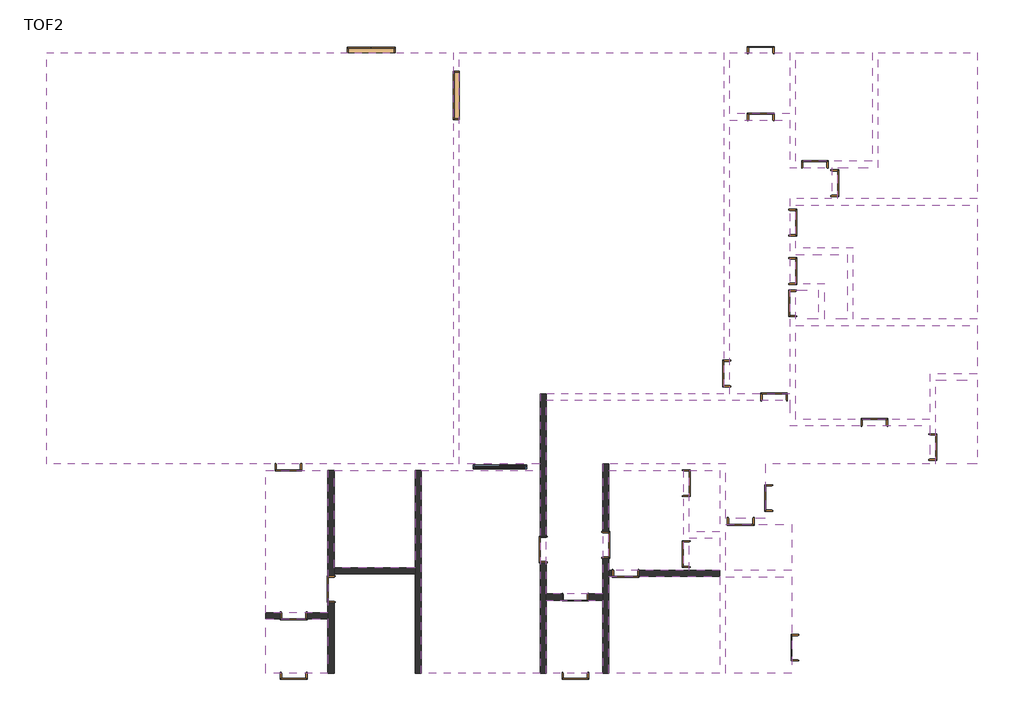
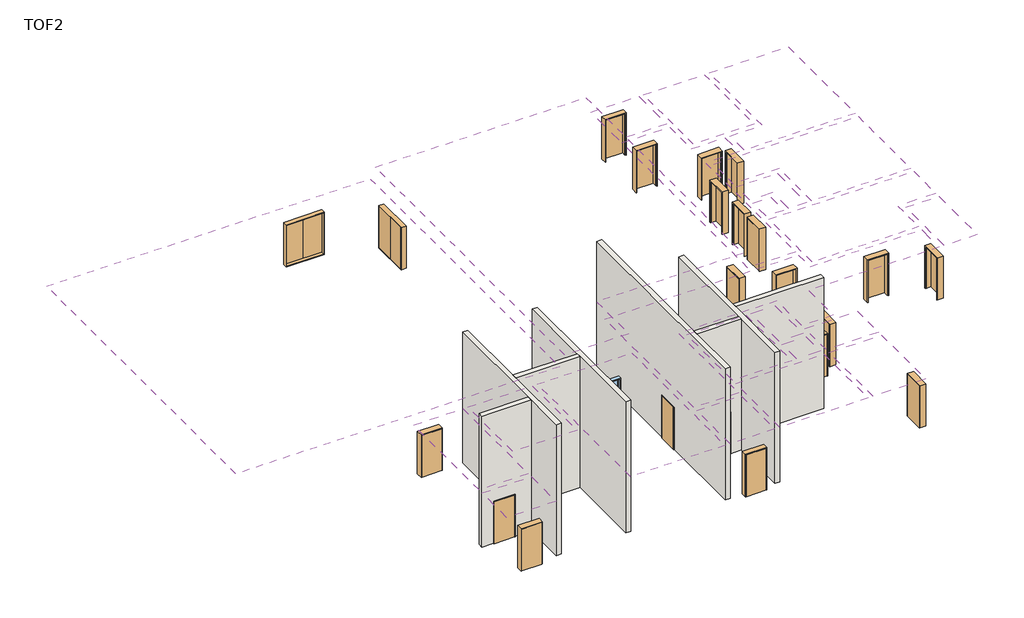
# One storey: 27 doors, 23 coverings, 8 walls, 1 window.
"""IFC4 building model written with IfcOpenShell, lengths in millimetres."""

import ifcopenshell
import ifcopenshell.guid

model = None  # the IFC model being written
_history = None  # IfcOwnerHistory: only IFC2X3 demands one
_inside = {}  # id of a spatial element -> (the spatial element, [elements in it])
_under = {}  # id of a project, library or spatial element -> (it, [spatial elements below it])
_declared = {}  # id of a project -> (the project, [libraries it declares])
_typed = {}  # id of a type object -> (the type object, [elements of that type])
_made_of = {}  # id of a material, layer set ... -> (it, [elements and type objects made of it])


def new_model(schema):
    """Start an empty IFC model of exactly this schema.

    Asked for "IFC4X3", IfcOpenShell would pick the latest addendum, in which some entities
    have other attributes; the version numbers below select the first issue.
    IFC2X3 requires an IfcOwnerHistory on every rooted entity: one is made here for all.
    """
    global model, _history
    if schema == "IFC4X3":
        model = ifcopenshell.file(schema_version=(4, 3, 0, 0))
    else:
        model = ifcopenshell.file(schema=schema)
    _inside.clear()
    _under.clear()
    _declared.clear()
    _typed.clear()
    _made_of.clear()
    _history = None
    if model.schema == "IFC2X3":
        org = make("IfcOrganization", Name="unknown")
        user = make(
            "IfcPersonAndOrganization",
            ThePerson=make("IfcPerson", FamilyName="unknown"),
            TheOrganization=org,
        )
        app = make(
            "IfcApplication",
            ApplicationDeveloper=org,
            Version="unknown",
            ApplicationFullName="unknown",
            ApplicationIdentifier="unknown",
        )
        _history = make(
            "IfcOwnerHistory",
            OwningUser=user,
            OwningApplication=app,
            ChangeAction="ADDED",
            CreationDate=0,
        )
    return model


def make(cls, **values):
    """One entity of the class cls with the attributes given. An attribute that is None is left unset."""
    return model.create_entity(
        cls, **{name: value for name, value in values.items() if value is not None}
    )


def rooted(cls, **values):
    """An entity with a GlobalId (a new one), such as an element, a storey or a relation."""
    return make(cls, GlobalId=ifcopenshell.guid.new(), OwnerHistory=_history, **values)


def si_unit(unit_type, name, prefix=None):
    """IfcSIUnit, for example si_unit("LENGTHUNIT", "METRE", prefix="MILLI")."""
    return make("IfcSIUnit", UnitType=unit_type, Prefix=prefix, Name=name)


def assignment(units):
    """IfcUnitAssignment: the units of a project."""
    return None if units is None else make("IfcUnitAssignment", Units=units)


def point(xyz):
    """IfcCartesianPoint."""
    return None if xyz is None else make("IfcCartesianPoint", Coordinates=xyz)


def direction(xyz):
    """IfcDirection."""
    return None if xyz is None else make("IfcDirection", DirectionRatios=xyz)


def frame(location, z_axis=None, x_axis=None):
    """IfcAxis2Placement3D, a coordinate frame: its origin and axes. An axis left out is left unset."""
    return make(
        "IfcAxis2Placement3D",
        Location=point(location),
        Axis=direction(z_axis),
        RefDirection=direction(x_axis),
    )


def origin():
    """The frame at (0, 0, 0) with its axes left unset."""
    return frame((0.0, 0.0, 0.0))


def origin_with_axes():
    """The frame at (0, 0, 0) with the z axis (0, 0, 1) and the x axis (1, 0, 0) written out."""
    return frame((0.0, 0.0, 0.0), z_axis=(0.0, 0.0, 1.0), x_axis=(1.0, 0.0, 0.0))


def place(relative_to, where):
    """IfcLocalPlacement: puts the frame where relative to a parent placement (None: the world)."""
    return make(
        "IfcLocalPlacement", PlacementRelTo=relative_to, RelativePlacement=where
    )


def context(
    kind, dimensions, precision=None, world=None, true_north=None, identifier=None
):
    """IfcGeometricRepresentationContext, for example the 3D "Model" context."""
    return make(
        "IfcGeometricRepresentationContext",
        ContextIdentifier=identifier,
        ContextType=kind,
        CoordinateSpaceDimension=dimensions,
        Precision=precision,
        WorldCoordinateSystem=world,
        TrueNorth=true_north,
    )


def project(units=None, contexts=None):
    """IfcProject with its units and contexts."""
    return rooted(
        "IfcProject",
        Name="project",
        RepresentationContexts=contexts,
        UnitsInContext=assignment(units),
    )


def spatial(cls, under=None, at=None, **own):
    """A site, building, storey or space (cls), placed at a placement, below another one or the project."""
    s = rooted(cls, ObjectPlacement=at, **own)
    if under is not None:
        _under.setdefault(under.id(), (under, []))[1].append(s)
    return s


def polyline(points):
    """IfcPolyline through the points."""
    return make("IfcPolyline", Points=[point(p) for p in points])


def outline(outer, holes=None, kind="AREA"):
    """IfcArbitraryClosedProfileDef: a profile drawn as a closed curve; with holes, ...WithVoids."""
    if holes is None:
        return make("IfcArbitraryClosedProfileDef", ProfileType=kind, OuterCurve=outer)
    return make(
        "IfcArbitraryProfileDefWithVoids",
        ProfileType=kind,
        OuterCurve=outer,
        InnerCurves=holes,
    )


def extrude(swept, where, along, depth):
    """IfcExtrudedAreaSolid: the profile swept, set in the frame where, extruded along a direction by depth."""
    return make(
        "IfcExtrudedAreaSolid",
        SweptArea=swept,
        Position=where,
        ExtrudedDirection=direction(along),
        Depth=depth,
    )


def faces_of(points, faces, orient=None, outer=None):
    """IfcFace entities. A face is a list of loops; a loop is a list of indices into points, from 0.

    orient and outer hold one flag for each loop. By default every Orientation is true, the
    first loop of a face is its IfcFaceOuterBound and the others are IfcFaceBound.
    """
    made = []
    for i, loops in enumerate(faces):
        bounds = []
        for j, loop in enumerate(loops):
            is_outer = j == 0 if outer is None else outer[i][j]
            bounds.append(
                make(
                    "IfcFaceOuterBound" if is_outer else "IfcFaceBound",
                    Bound=make("IfcPolyLoop", Polygon=[points[k] for k in loop]),
                    Orientation=True if orient is None else orient[i][j],
                )
            )
        made.append(make("IfcFace", Bounds=bounds))
    return made


def faceted_brep(points, faces, orient=None, outer=None, voids=None):
    """IfcFacetedBrep: a solid bounded by flat faces; with voids (closed shells), ...WithVoids."""
    shared = [point(p) for p in points]
    hull = make("IfcClosedShell", CfsFaces=faces_of(shared, faces, orient, outer))
    if voids is None:
        return make("IfcFacetedBrep", Outer=hull)
    return make(
        "IfcFacetedBrepWithVoids",
        Outer=hull,
        Voids=[
            make(cls, CfsFaces=faces_of(shared, fs, o, b)) for cls, fs, o, b in voids
        ],
    )


def shape(context_of_items, identifier, shape_type, items):
    """IfcShapeRepresentation: the items that make up one representation, for example the "Body"."""
    return make(
        "IfcShapeRepresentation",
        ContextOfItems=context_of_items,
        RepresentationIdentifier=identifier,
        RepresentationType=shape_type,
        Items=items,
    )


def source(mapping_origin, context_of_items, identifier, shape_type, items):
    """IfcRepresentationMap: a shape defined once, which mapped items show again and again."""
    return make(
        "IfcRepresentationMap",
        MappingOrigin=mapping_origin,
        MappedRepresentation=shape(context_of_items, identifier, shape_type, items),
    )


def transform(
    local_origin,
    x_axis=None,
    y_axis=None,
    z_axis=None,
    scale=None,
    scale2=None,
    scale3=None,
    uniform=True,
):
    """IfcCartesianTransformationOperator3D, or its non-uniform kind. x_axis, y_axis, z_axis: its Axis1, 2, 3."""
    if uniform:
        return make(
            "IfcCartesianTransformationOperator3D",
            Axis1=direction(x_axis),
            Axis2=direction(y_axis),
            LocalOrigin=point(local_origin),
            Scale=scale,
            Axis3=direction(z_axis),
        )
    return make(
        "IfcCartesianTransformationOperator3DnonUniform",
        Axis1=direction(x_axis),
        Axis2=direction(y_axis),
        LocalOrigin=point(local_origin),
        Scale=scale,
        Axis3=direction(z_axis),
        Scale2=scale2,
        Scale3=scale3,
    )


def mapped(mapping_source, mapping_target):
    """IfcMappedItem: shows the shape of a source again, moved by a transform."""
    return make(
        "IfcMappedItem", MappingSource=mapping_source, MappingTarget=mapping_target
    )


def made_of(thing, what):
    """Note that an element or type object is made of a material, layer set ...; save() writes the relation."""
    if what is not None:
        _made_of.setdefault(what.id(), (what, []))[1].append(thing)
    return thing


def element(
    cls,
    number,
    at=None,
    inside=None,
    cuts=None,
    type_object=None,
    material=None,
    context=None,
    identifier="Body",
    shape_type=None,
    held_by="IfcProductDefinitionShape",
    body=None,
    shapes=None,
    **own,
):
    """One element of the class cls, such as IfcWall. Its Tag is "e" and its number.

    at: its placement. inside: the storey or other place that contains it. cuts: it is an
    opening in that element (IfcRelVoidsElement). A single representation is given by context,
    identifier, shape_type and body (its items); several are given by shapes. held_by: the class
    of the entity that holds the representations. save() writes the other relations.
    """
    e = rooted(cls, Tag="e%d" % number, ObjectPlacement=at, **own)
    if body is not None:
        shapes = [shape(context, identifier, shape_type, body)]
    if shapes is not None:
        e.Representation = make(held_by, Representations=shapes)
    if inside is not None:
        _inside.setdefault(inside.id(), (inside, []))[1].append(e)
    if cuts is not None:
        rooted(
            "IfcRelVoidsElement", RelatingBuildingElement=cuts, RelatedOpeningElement=e
        )
    if type_object is not None:
        _typed.setdefault(type_object.id(), (type_object, []))[1].append(e)
    return made_of(e, material)


def aggregate(whole, parts):
    """IfcRelAggregates: a whole, such as a stair, and the parts it consists of."""
    return rooted("IfcRelAggregates", RelatingObject=whole, RelatedObjects=parts)


def save(model, path):
    """Write the relations noted so far, then the file.

    IfcRelAggregates (storeys below a building ...), IfcRelContainedInSpatialStructure (elements
    in a storey), IfcRelDefinesByType, IfcRelAssociatesMaterial and IfcRelDeclares: one each for
    every whole, place, type object, material and project.
    """
    for whole, parts in _under.values():
        aggregate(whole, parts)
    for where, things in _inside.values():
        rooted(
            "IfcRelContainedInSpatialStructure",
            RelatedElements=things,
            RelatingStructure=where,
        )
    for kind, things in _typed.values():
        rooted("IfcRelDefinesByType", RelatedObjects=things, RelatingType=kind)
    for what, things in _made_of.values():
        rooted("IfcRelAssociatesMaterial", RelatedObjects=things, RelatingMaterial=what)
    for by, libraries in _declared.values():
        rooted("IfcRelDeclares", RelatingContext=by, RelatedDefinitions=libraries)
    model.write(path)


def double_door_steel_22a565f0(model_context):
    return source(origin(), model_context, "Body", "SolidModel", [
        extrude(outline(polyline([(880.0, 60.0), (0.0, 60.0), (0.0, 100.0), (880.0, 100.0), (880.0, 60.0)])), frame((0.0, 0.0, 20.0), z_axis=(0.0, 0.0, 1.0), x_axis=(1.0, 0.0, 0.0)), (0.0, 0.0, 1.0), 2060.0),
        extrude(outline(polyline([(0.0, 60.0), (-880.0, 60.0), (-880.0, 100.0), (0.0, 100.0), (0.0, 60.0)])), frame((0.0, 0.0, 20.0), z_axis=(0.0, 0.0, 1.0), x_axis=(1.0, 0.0, 0.0)), (0.0, 0.0, 1.0), 2060.0),
        faceted_brep([(900.0, -100.0, 2100.0), (900.0, 100.0, 2100.0), (-900.0, 100.0, 2100.0), (-900.0, -100.0, 2100.0), (865.0, 60.0, 2065.0), (865.0, -100.0, 2065.0), (-865.0, -100.0, 2065.0), (-865.0, 60.0, 2065.0), (880.0, 100.0, 2080.0), (880.0, 60.0, 2080.0), (-880.0, 60.0, 2080.0), (-880.0, 100.0, 2080.0), (-900.0, 100.0, 0.0), (-900.0, -100.0, 0.0), (-865.0, -100.0, 35.0), (-865.0, 60.0, 35.0), (-880.0, 60.0, 20.0), (-880.0, 100.0, 20.0), (900.0, 100.0, 0.0), (880.0, 100.0, 20.0), (900.0, -100.0, 0.0), (865.0, -100.0, 35.0), (865.0, 60.0, 35.0), (880.0, 60.0, 20.0)], [[[0, 1, 2, 3]], [[4, 5, 6, 7]], [[8, 9, 10, 11]], [[3, 2, 12, 13]], [[7, 6, 14, 15]], [[11, 10, 16, 17]], [[18, 12, 2, 1], [8, 11, 17, 19]], [[13, 12, 18, 20]], [[0, 3, 13, 20], [21, 14, 6, 5]], [[15, 14, 21, 22]], [[23, 16, 10, 9], [4, 7, 15, 22]], [[17, 16, 23, 19]], [[20, 18, 1, 0]], [[22, 21, 5, 4]], [[19, 23, 9, 8]]]),
    ])


def double_door_steel_ece7098f(model_context):
    return source(origin(), model_context, "Body", "SolidModel", [
        extrude(outline(polyline([(880.0, 77.0), (0.0, 77.0), (0.0, 117.0), (880.0, 117.0), (880.0, 77.0)])), frame((0.0, 0.0, 20.0), z_axis=(0.0, 0.0, 1.0), x_axis=(1.0, 0.0, 0.0)), (0.0, 0.0, 1.0), 2060.0),
        extrude(outline(polyline([(0.0, 77.0), (-880.0, 77.0), (-880.0, 117.0), (0.0, 117.0), (0.0, 77.0)])), frame((0.0, 0.0, 20.0), z_axis=(0.0, 0.0, 1.0), x_axis=(1.0, 0.0, 0.0)), (0.0, 0.0, 1.0), 2060.0),
        faceted_brep([(900.0, -117.0, 2100.0), (900.0, 117.0, 2100.0), (-900.0, 117.0, 2100.0), (-900.0, -117.0, 2100.0), (865.0, 77.0, 2065.0), (865.0, -117.0, 2065.0), (-865.0, -117.0, 2065.0), (-865.0, 77.0, 2065.0), (880.0, 117.0, 2080.0), (880.0, 77.0, 2080.0), (-880.0, 77.0, 2080.0), (-880.0, 117.0, 2080.0), (-900.0, 117.0, 0.0), (-900.0, -117.0, 0.0), (-865.0, -117.0, 35.0), (-865.0, 77.0, 35.0), (-880.0, 77.0, 20.0), (-880.0, 117.0, 20.0), (900.0, 117.0, 0.0), (880.0, 117.0, 20.0), (900.0, -117.0, 0.0), (865.0, -117.0, 35.0), (865.0, 77.0, 35.0), (880.0, 77.0, 20.0)], [[[0, 1, 2, 3]], [[4, 5, 6, 7]], [[8, 9, 10, 11]], [[3, 2, 12, 13]], [[7, 6, 14, 15]], [[11, 10, 16, 17]], [[18, 12, 2, 1], [8, 11, 17, 19]], [[13, 12, 18, 20]], [[0, 3, 13, 20], [21, 14, 6, 5]], [[15, 14, 21, 22]], [[23, 16, 10, 9], [4, 7, 15, 22]], [[17, 16, 23, 19]], [[20, 18, 1, 0]], [[22, 21, 5, 4]], [[19, 23, 9, 8]]]),
    ])


def single_door_steel_02f153ad(model_context):
    return source(origin(), model_context, "Body", "SolidModel", [
        extrude(outline(polyline([(470.0, -130.0), (-470.0, -130.0), (-470.0, -95.0), (470.0, -95.0), (470.0, -130.0)])), origin_with_axes(), (0.0, 0.0, 1.0), 2070.0),
        faceted_brep([(470.0, -130.0, 0.0), (470.0, -95.0, 0.0), (450.0, -95.0, 0.0), (450.0, 95.0, 0.0), (470.0, 95.0, 0.0), (470.0, 130.0, 0.0), (500.0, 130.0, 0.0), (500.0, -130.0, 0.0), (500.0, -130.0, 2100.0), (-500.0, -130.0, 2100.0), (-500.0, -130.0, 0.0), (-470.0, -130.0, 0.0), (-470.0, -130.0, 2070.0), (470.0, -130.0, 2070.0), (500.0, 130.0, 2100.0), (470.0, 130.0, 2070.0), (-470.0, 130.0, 2070.0), (-470.0, 130.0, 0.0), (-500.0, 130.0, 0.0), (-500.0, 130.0, 2100.0), (470.0, 95.0, 2070.0), (450.0, 95.0, 2050.0), (-450.0, 95.0, 2050.0), (-450.0, 95.0, 0.0), (-470.0, 95.0, 0.0), (-470.0, 95.0, 2070.0), (450.0, -95.0, 2050.0), (470.0, -95.0, 2070.0), (-470.0, -95.0, 2070.0), (-470.0, -95.0, 0.0), (-450.0, -95.0, 0.0), (-450.0, -95.0, 2050.0)], [[[0, 1, 2, 3, 4, 5, 6, 7]], [[7, 8, 9, 10, 11, 12, 13, 0]], [[6, 14, 8, 7]], [[5, 15, 16, 17, 18, 19, 14, 6]], [[4, 20, 15, 5]], [[3, 21, 22, 23, 24, 25, 20, 4]], [[2, 26, 21, 3]], [[1, 27, 28, 29, 30, 31, 26, 2]], [[0, 13, 27, 1]], [[12, 11, 29, 28]], [[11, 10, 18, 17, 24, 23, 30, 29]], [[19, 18, 10, 9]], [[25, 24, 17, 16]], [[31, 30, 23, 22]], [[14, 19, 9, 8]], [[20, 25, 16, 15]], [[26, 31, 22, 21]], [[13, 12, 28, 27]]]),
    ])


def single_door_steel_4a6c7de9(model_context):
    return source(origin(), model_context, "Body", "SolidModel", [
        extrude(outline(polyline([(470.0, 130.0), (470.0, 95.0), (-470.0, 95.0), (-470.0, 130.0), (470.0, 130.0)])), origin_with_axes(), (0.0, 0.0, 1.0), 2070.0),
        faceted_brep([(470.0, 130.0, 0.0), (500.0, 130.0, 0.0), (500.0, -130.0, 0.0), (470.0, -130.0, 0.0), (470.0, -95.0, 0.0), (450.0, -95.0, 0.0), (450.0, 95.0, 0.0), (470.0, 95.0, 0.0), (470.0, 130.0, 2070.0), (-470.0, 130.0, 2070.0), (-470.0, 130.0, 0.0), (-500.0, 130.0, 0.0), (-500.0, 130.0, 2100.0), (500.0, 130.0, 2100.0), (500.0, -130.0, 2100.0), (-500.0, -130.0, 2100.0), (-500.0, -130.0, 0.0), (-470.0, -130.0, 0.0), (-470.0, -130.0, 2070.0), (470.0, -130.0, 2070.0), (470.0, -95.0, 2070.0), (-470.0, -95.0, 2070.0), (-470.0, -95.0, 0.0), (-450.0, -95.0, 0.0), (-450.0, -95.0, 2050.0), (450.0, -95.0, 2050.0), (450.0, 95.0, 2050.0), (-450.0, 95.0, 2050.0), (-450.0, 95.0, 0.0), (-470.0, 95.0, 0.0), (-470.0, 95.0, 2070.0), (470.0, 95.0, 2070.0)], [[[0, 1, 2, 3, 4, 5, 6, 7]], [[1, 0, 8, 9, 10, 11, 12, 13]], [[2, 1, 13, 14]], [[3, 2, 14, 15, 16, 17, 18, 19]], [[4, 3, 19, 20]], [[5, 4, 20, 21, 22, 23, 24, 25]], [[6, 5, 25, 26]], [[7, 6, 26, 27, 28, 29, 30, 31]], [[0, 7, 31, 8]], [[9, 30, 29, 10]], [[10, 29, 28, 23, 22, 17, 16, 11]], [[15, 12, 11, 16]], [[21, 18, 17, 22]], [[27, 24, 23, 28]], [[14, 13, 12, 15]], [[20, 19, 18, 21]], [[26, 25, 24, 27]], [[8, 31, 30, 9]]]),
    ])


def single_door_steel_29c29026(model_context):
    return source(origin(), model_context, "Body", "SolidModel", [
        extrude(outline(polyline([(470.0, -147.0), (-470.0, -147.0), (-470.0, -112.0), (470.0, -112.0), (470.0, -147.0)])), origin_with_axes(), (0.0, 0.0, 1.0), 2070.0),
        faceted_brep([(470.0, -147.0, 0.0), (470.0, -112.0, 0.0), (450.0, -112.0, 0.0), (450.0, 112.0, 0.0), (470.0, 112.0, 0.0), (470.0, 147.0, 0.0), (500.0, 147.0, 0.0), (500.0, -147.0, 0.0), (500.0, -147.0, 2100.0), (-500.0, -147.0, 2100.0), (-500.0, -147.0, 0.0), (-470.0, -147.0, 0.0), (-470.0, -147.0, 2070.0), (470.0, -147.0, 2070.0), (500.0, 147.0, 2100.0), (470.0, 147.0, 2070.0), (-470.0, 147.0, 2070.0), (-470.0, 147.0, 0.0), (-500.0, 147.0, 0.0), (-500.0, 147.0, 2100.0), (470.0, 112.0, 2070.0), (450.0, 112.0, 2050.0), (-450.0, 112.0, 2050.0), (-450.0, 112.0, 0.0), (-470.0, 112.0, 0.0), (-470.0, 112.0, 2070.0), (450.0, -112.0, 2050.0), (470.0, -112.0, 2070.0), (-470.0, -112.0, 2070.0), (-470.0, -112.0, 0.0), (-450.0, -112.0, 0.0), (-450.0, -112.0, 2050.0)], [[[0, 1, 2, 3, 4, 5, 6, 7]], [[7, 8, 9, 10, 11, 12, 13, 0]], [[6, 14, 8, 7]], [[5, 15, 16, 17, 18, 19, 14, 6]], [[4, 20, 15, 5]], [[3, 21, 22, 23, 24, 25, 20, 4]], [[2, 26, 21, 3]], [[1, 27, 28, 29, 30, 31, 26, 2]], [[0, 13, 27, 1]], [[12, 11, 29, 28]], [[11, 10, 18, 17, 24, 23, 30, 29]], [[19, 18, 10, 9]], [[25, 24, 17, 16]], [[31, 30, 23, 22]], [[14, 19, 9, 8]], [[20, 25, 16, 15]], [[26, 31, 22, 21]], [[13, 12, 28, 27]]]),
    ])


def single_door_steel_aae97da1(model_context):
    return source(origin(), model_context, "Body", "SolidModel", [
        extrude(outline(polyline([(470.0, 147.0), (470.0, 112.0), (-470.0, 112.0), (-470.0, 147.0), (470.0, 147.0)])), origin_with_axes(), (0.0, 0.0, 1.0), 2070.0),
        faceted_brep([(470.0, 147.0, 0.0), (500.0, 147.0, 0.0), (500.0, -147.0, 0.0), (470.0, -147.0, 0.0), (470.0, -112.0, 0.0), (450.0, -112.0, 0.0), (450.0, 112.0, 0.0), (470.0, 112.0, 0.0), (470.0, 147.0, 2070.0), (-470.0, 147.0, 2070.0), (-470.0, 147.0, 0.0), (-500.0, 147.0, 0.0), (-500.0, 147.0, 2100.0), (500.0, 147.0, 2100.0), (500.0, -147.0, 2100.0), (-500.0, -147.0, 2100.0), (-500.0, -147.0, 0.0), (-470.0, -147.0, 0.0), (-470.0, -147.0, 2070.0), (470.0, -147.0, 2070.0), (470.0, -112.0, 2070.0), (-470.0, -112.0, 2070.0), (-470.0, -112.0, 0.0), (-450.0, -112.0, 0.0), (-450.0, -112.0, 2050.0), (450.0, -112.0, 2050.0), (450.0, 112.0, 2050.0), (-450.0, 112.0, 2050.0), (-450.0, 112.0, 0.0), (-470.0, 112.0, 0.0), (-470.0, 112.0, 2070.0), (470.0, 112.0, 2070.0)], [[[0, 1, 2, 3, 4, 5, 6, 7]], [[1, 0, 8, 9, 10, 11, 12, 13]], [[2, 1, 13, 14]], [[3, 2, 14, 15, 16, 17, 18, 19]], [[4, 3, 19, 20]], [[5, 4, 20, 21, 22, 23, 24, 25]], [[6, 5, 25, 26]], [[7, 6, 26, 27, 28, 29, 30, 31]], [[0, 7, 31, 8]], [[9, 30, 29, 10]], [[10, 29, 28, 23, 22, 17, 16, 11]], [[15, 12, 11, 16]], [[21, 18, 17, 22]], [[27, 24, 23, 28]], [[14, 13, 12, 15]], [[20, 19, 18, 21]], [[26, 25, 24, 27]], [[8, 31, 30, 9]]]),
    ])


def sliding_window_5e64f0fd(model_context):
    return source(origin(), model_context, "Body", "SolidModel", [
        extrude(outline(polyline([(920.0, 27.5), (25.0, 27.5), (25.0, 32.5), (920.0, 32.5), (920.0, 27.5)])), frame((0.0, 0.0, 680.0), z_axis=(0.0, 0.0, 1.0), x_axis=(1.0, 0.0, 0.0)), (0.0, 0.0, 1.0), 840.0),
        extrude(outline(polyline([(-25.0, -32.5), (-920.0, -32.5), (-920.0, -27.5), (-25.0, -27.5), (-25.0, -32.5)])), frame((0.0, 0.0, 680.0), z_axis=(0.0, 0.0, 1.0), x_axis=(1.0, 0.0, 0.0)), (0.0, 0.0, 1.0), 840.0),
        extrude(outline(polyline([(630.0, -970.0), (630.0, 25.0), (1570.0, 25.0), (1570.0, -970.0), (630.0, -970.0)]), holes=[polyline([(1520.0, -920.0), (1520.0, -25.0), (680.0, -25.0), (680.0, -920.0), (1520.0, -920.0)])]), frame((0.0, -55.0, 0.0), z_axis=(0.0, 1.0, 0.0), x_axis=(0.0, 0.0, 1.0)), (0.0, 0.0, 1.0), 47.5),
        extrude(outline(polyline([(630.0, -25.0), (630.0, 970.0), (1570.0, 970.0), (1570.0, -25.0), (630.0, -25.0)]), holes=[polyline([(1520.0, 25.0), (1520.0, 920.0), (680.0, 920.0), (680.0, 25.0), (1520.0, 25.0)])]), frame((0.0, 7.5, 0.0), z_axis=(0.0, 1.0, 0.0), x_axis=(0.0, 0.0, 1.0)), (0.0, 0.0, 1.0), 45.0),
        faceted_brep([(-1000.0, 75.0, 1600.0), (-1000.0, 75.0, 600.0), (-1000.0, -75.0, 600.0), (-1000.0, -75.0, 1600.0), (1000.0, 75.0, 1600.0), (1000.0, 75.0, 600.0), (950.0, 75.0, 650.0), (950.0, 75.0, 1550.0), (-950.0, 75.0, 1550.0), (-950.0, 75.0, 650.0), (1000.0, -75.0, 600.0), (1000.0, -75.0, 1600.0), (-950.0, -75.0, 1550.0), (950.0, -75.0, 1550.0), (950.0, -75.0, 650.0), (-950.0, -75.0, 650.0), (950.0, 55.0, 650.0), (950.0, 55.0, 1550.0), (-950.0, 55.0, 1550.0), (-950.0, 55.0, 1570.0), (-950.0, 5.0, 1570.0), (-950.0, 5.0, 1550.0), (-950.0, -5.0, 1550.0), (-950.0, -5.0, 650.0), (-950.0, 5.0, 650.0), (-950.0, 5.0, 630.0), (-950.0, 55.0, 630.0), (-950.0, 55.0, 650.0), (950.0, -5.0, 650.0), (950.0, 5.0, 650.0), (950.0, -5.0, 630.0), (950.0, -55.0, 630.0), (950.0, -55.0, 650.0), (950.0, -55.0, 1550.0), (950.0, -55.0, 1570.0), (950.0, -5.0, 1570.0), (950.0, -5.0, 1550.0), (950.0, 5.0, 1550.0), (970.0, 5.0, 1570.0), (970.0, 5.0, 630.0), (-970.0, -5.0, 1570.0), (-970.0, -5.0, 630.0), (970.0, 55.0, 1570.0), (970.0, 55.0, 630.0), (-970.0, -55.0, 630.0), (-950.0, -55.0, 1550.0), (-950.0, -55.0, 650.0), (-970.0, -55.0, 1570.0)], [[[0, 1, 2, 3]], [[4, 5, 1, 0], [6, 7, 8, 9]], [[1, 5, 10, 2]], [[10, 11, 3, 2], [12, 13, 14, 15]], [[7, 6, 16, 17]], [[9, 8, 18, 19, 20, 21, 22, 23, 24, 25, 26, 27]], [[16, 6, 9, 27]], [[5, 4, 11, 10]], [[28, 29, 24, 23]], [[28, 30, 31, 32, 14, 13, 33, 34, 35, 36, 37, 29]], [[29, 37, 21, 20, 38, 39, 25, 24]], [[40, 41, 30, 28, 23, 22, 36, 35]], [[39, 38, 42, 43]], [[39, 43, 26, 25]], [[43, 42, 19, 18, 17, 16, 27, 26]], [[41, 44, 31, 30]], [[45, 46, 32, 31, 44, 47, 34, 33]], [[46, 15, 14, 32]], [[12, 15, 46, 45]], [[47, 44, 41, 40]], [[3, 11, 4, 0]], [[7, 17, 18, 8]], [[37, 36, 22, 21]], [[42, 38, 20, 19]], [[12, 45, 33, 13]], [[47, 40, 35, 34]]]),
    ])


model = new_model("IFC4")

# Units and contexts
model_context = context("Model", 3, world=origin())
ifc_project = project(units=[si_unit("LENGTHUNIT", "METRE", prefix="MILLI")], contexts=[model_context])

# Site, building, storey
site = spatial("IfcSite", under=ifc_project)
building = spatial("IfcBuilding", under=site)
storey = spatial("IfcBuildingStorey", under=building, Name="TOF2", Elevation=1149.9618634)

# Coverings
placement = place(None, origin())
element("IfcCovering", 1, ObjectType="H_CE_AR_B09_Acoustic Ceiling_T Bar_600x600x9T", at=placement, inside=storey, context=model_context, shape_type="SweptSolid", body=[
    extrude(outline(polyline([(18112.0, 8416.5208589), (18112.0, 23799.5208589), (33303.0, 23799.5208589), (33303.0, 8416.5208589), (18112.0, 8416.5208589)])), frame((0.0, 0.0, 4149.9618634), z_axis=(0.0, 0.0, 1.0), x_axis=(1.0, 0.0, 0.0)), (0.0, 0.0, 1.0), 9.0),
])
element("IfcCovering", 2, ObjectType="H_CE_AR_B09_Acoustic Ceiling_T Bar_600x600x9T", at=placement, inside=storey, context=model_context, shape_type="SweptSolid", body=[
    extrude(outline(polyline([(33537.0, 8416.5208589), (33537.0, 23799.5208589), (43413.0, 23799.5208589), (43413.0, 11036.5208589), (36553.0, 11036.5208589), (36553.0, 8416.5208589), (33537.0, 8416.5208589)])), frame((0.0, 0.0, 4649.9618634), z_axis=(0.0, 0.0, 1.0), x_axis=(1.0, 0.0, 0.0)), (0.0, 0.0, 1.0), 9.0),
])
element("IfcCovering", 3, ObjectType="H_CE_AR_B09_Acoustic Ceiling_T Bar_600x600x9T", at=placement, inside=storey, context=model_context, shape_type="SweptSolid", body=[
    extrude(outline(polyline([(43647.0, 23799.5208589), (45883.0, 23799.5208589), (45883.0, 21511.5208589), (43647.0, 21511.5208589), (43647.0, 23799.5208589)])), frame((0.0, 0.0, 3849.9618634), z_axis=(0.0, 0.0, 1.0), x_axis=(1.0, 0.0, 0.0)), (0.0, 0.0, 1.0), 9.0),
])
element("IfcCovering", 4, ObjectType="H_CE_AR_B09_Acoustic Ceiling_T Bar_600x600x9T", at=placement, inside=storey, context=model_context, shape_type="SweptSolid", body=[
    extrude(outline(polyline([(46117.0, 23799.5208589), (48963.0, 23799.5208589), (48963.0, 19736.5208589), (46117.0, 19736.5208589), (46117.0, 23799.5208589)])), frame((0.0, 0.0, 3849.9618634), z_axis=(0.0, 0.0, 1.0), x_axis=(1.0, 0.0, 0.0)), (0.0, 0.0, 1.0), 9.0),
])
element("IfcCovering", 5, ObjectType="H_CE_AR_B09_Acoustic Ceiling_T Bar_600x600x9T", at=placement, inside=storey, context=model_context, shape_type="SweptSolid", body=[
    extrude(outline(polyline([(49197.0, 23799.5208589), (52900.0, 23799.5208589), (52900.0, 18336.5208589), (47687.0, 18336.5208589), (47687.0, 19502.5208589), (49197.0, 19502.5208589), (49197.0, 23799.5208589)])), frame((0.0, 0.0, 3849.9618634), z_axis=(0.0, 0.0, 1.0), x_axis=(1.0, 0.0, 0.0)), (0.0, 0.0, 1.0), 9.0),
])
element("IfcCovering", 6, ObjectType="H_CE_AR_B09_Acoustic Ceiling_T Bar_600x600x9T", at=placement, inside=storey, context=model_context, shape_type="SweptSolid", body=[
    extrude(outline(polyline([(45883.0, 18336.5208589), (45883.0, 11036.5208589), (43647.0, 11036.5208589), (43647.0, 21277.5208589), (45883.0, 21277.5208589), (45883.0, 19502.5208589), (47453.0, 19502.5208589), (47453.0, 18336.5208589), (45883.0, 18336.5208589)])), frame((0.0, 0.0, 3849.9618634), z_axis=(0.0, 0.0, 1.0), x_axis=(1.0, 0.0, 0.0)), (0.0, 0.0, 1.0), 9.0),
])
element("IfcCovering", 7, ObjectType="H_CE_AR_B09_Acoustic Ceiling_T Bar_600x600x9T", at=placement, inside=storey, context=model_context, shape_type="SweptSolid", body=[
    extrude(outline(polyline([(52900.0, 18102.5208589), (52900.0, 13836.5208589), (48262.0, 13836.5208589), (48262.0, 16486.5208589), (46117.0, 16486.5208589), (46117.0, 18102.5208589), (52900.0, 18102.5208589)])), frame((0.0, 0.0, 3849.9618634), z_axis=(0.0, 0.0, 1.0), x_axis=(1.0, 0.0, 0.0)), (0.0, 0.0, 1.0), 9.0),
])
element("IfcCovering", 8, ObjectType="H_CE_AR_B09_Acoustic Ceiling_T Bar_600x600x9T", at=placement, inside=storey, context=model_context, shape_type="SweptSolid", body=[
    extrude(outline(polyline([(47187.0, 15151.5208589), (46117.0, 15151.5208589), (46117.0, 16252.5208589), (48028.0, 16252.5208589), (48028.0, 13836.5208589), (47187.0, 13836.5208589), (47187.0, 15151.5208589)])), frame((0.0, 0.0, 3849.9618634), z_axis=(0.0, 0.0, 1.0), x_axis=(1.0, 0.0, 0.0)), (0.0, 0.0, 1.0), 9.0),
])
element("IfcCovering", 9, ObjectType="H_CE_AR_B09_Acoustic Ceiling_T Bar_600x600x9T", at=placement, inside=storey, context=model_context, shape_type="SweptSolid", body=[
    extrude(outline(polyline([(46953.0, 13836.5208589), (46117.0, 13836.5208589), (46117.0, 14917.5208589), (46953.0, 14917.5208589), (46953.0, 13836.5208589)])), frame((0.0, 0.0, 3849.9618634), z_axis=(0.0, 0.0, 1.0), x_axis=(1.0, 0.0, 0.0)), (0.0, 0.0, 1.0), 9.0),
])
element("IfcCovering", 10, ObjectType="H_CE_AR_B09_Acoustic Ceiling_T Bar_600x600x9T", at=placement, inside=storey, context=model_context, shape_type="SweptSolid", body=[
    extrude(outline(polyline([(52900.0, 13602.5208589), (52900.0, 11786.5208589), (51113.0, 11786.5208589), (51113.0, 10086.5208589), (46117.0, 10086.5208589), (46117.0, 13602.5208589), (52900.0, 13602.5208589)])), frame((0.0, 0.0, 3849.9618634), z_axis=(0.0, 0.0, 1.0), x_axis=(1.0, 0.0, 0.0)), (0.0, 0.0, 1.0), 9.0),
])
element("IfcCovering", 11, ObjectType="H_CE_AR_B09_Acoustic Ceiling_T Bar_600x600x9T", at=placement, inside=storey, context=model_context, shape_type="SweptSolid", body=[
    extrude(outline(polyline([(52900.0, 11552.5208589), (52900.0, 8411.5208589), (51347.0, 8411.5208589), (51347.0, 11552.5208589), (52900.0, 11552.5208589)])), frame((0.0, 0.0, 3849.9618634), z_axis=(0.0, 0.0, 1.0), x_axis=(1.0, 0.0, 0.0)), (0.0, 0.0, 1.0), 9.0),
])
element("IfcCovering", 12, ObjectType="H_CE_AR_B09_Acoustic Ceiling_T Bar_600x600x9T", at=placement, inside=storey, context=model_context, shape_type="SweptSolid", body=[
    extrude(outline(polyline([(38888.0, 3555.8249516), (36787.0, 3555.8249516), (36787.0, 10802.5208589), (45883.0, 10802.5208589), (45883.0, 9852.5208589), (51113.0, 9852.5208589), (51113.0, 8411.5208589), (44978.0, 8411.5208589), (44978.0, 6390.8249516), (43497.0, 6390.8249516), (43497.0, 8416.5208589), (38888.0, 8416.5208589), (38888.0, 3555.8249516)])), frame((0.0, 0.0, 3849.9618634), z_axis=(0.0, 0.0, 1.0), x_axis=(1.0, 0.0, 0.0)), (0.0, 0.0, 1.0), 9.0),
])
element("IfcCovering", 13, ObjectType="H_CE_AR_B09_Acoustic Ceiling_T Bar_600x600x9T", at=placement, inside=storey, context=model_context, shape_type="SweptSolid", body=[
    extrude(outline(polyline([(45963.0, 4196.8249516), (45963.0, 599.5208589), (43497.0, 599.5208589), (43497.0, 4196.8249516), (45963.0, 4196.8249516)])), frame((0.0, 0.0, 3849.9618634), z_axis=(0.0, 0.0, 1.0), x_axis=(1.0, 0.0, 0.0)), (0.0, 0.0, 1.0), 9.0),
])
element("IfcCovering", 14, ObjectType="H_CE_AR_B09_Acoustic Ceiling_T Bar_600x600x9T", at=placement, inside=storey, context=model_context, shape_type="SweptSolid", body=[
    extrude(outline(polyline([(45963.0, 4430.8249516), (43497.0, 4430.8249516), (43497.0, 6156.8249516), (45963.0, 6156.8249516), (45963.0, 4430.8249516)])), frame((0.0, 0.0, 3849.9618634), z_axis=(0.0, 0.0, 1.0), x_axis=(1.0, 0.0, 0.0)), (0.0, 0.0, 1.0), 9.0),
])
element("IfcCovering", 15, ObjectType="H_CE_AR_B09_Acoustic Ceiling_T Bar_600x600x9T", at=placement, inside=storey, context=model_context, shape_type="SweptSolid", body=[
    extrude(outline(polyline([(43263.0, 5652.5208589), (43263.0, 4440.8249516), (42137.0, 4440.8249516), (42137.0, 5652.5208589), (43263.0, 5652.5208589)])), frame((0.0, 0.0, 3849.9618634), z_axis=(0.0, 0.0, 1.0), x_axis=(1.0, 0.0, 0.0)), (0.0, 0.0, 1.0), 9.0),
])
element("IfcCovering", 16, ObjectType="H_CE_AR_B09_Acoustic Ceiling_T Bar_600x600x9T", at=placement, inside=storey, context=model_context, shape_type="SweptSolid", body=[
    extrude(outline(polyline([(42137.0, 5886.5208589), (42137.0, 8182.5208589), (43263.0, 8182.5208589), (43263.0, 5886.5208589), (42137.0, 5886.5208589)])), frame((0.0, 0.0, 3849.9618634), z_axis=(0.0, 0.0, 1.0), x_axis=(1.0, 0.0, 0.0)), (0.0, 0.0, 1.0), 9.0),
])
element("IfcCovering", 17, ObjectType="H_CE_AR_B09_Acoustic Ceiling_T Bar_600x600x9T", at=placement, inside=storey, context=model_context, shape_type="SweptSolid", body=[
    extrude(outline(polyline([(39122.0, 4440.8249516), (39122.0, 8182.5208589), (41903.0, 8182.5208589), (41903.0, 4440.8249516), (39122.0, 4440.8249516)])), frame((0.0, 0.0, 3849.9618634), z_axis=(0.0, 0.0, 1.0), x_axis=(1.0, 0.0, 0.0)), (0.0, 0.0, 1.0), 9.0),
])
element("IfcCovering", 18, ObjectType="H_CE_AR_B09_Acoustic Ceiling_T Bar_600x600x9T", at=placement, inside=storey, context=model_context, shape_type="SweptSolid", body=[
    extrude(outline(polyline([(43263.0, 4206.8249516), (43263.0, 599.5208589), (39122.0, 599.5208589), (39122.0, 4206.8249516), (43263.0, 4206.8249516)])), frame((0.0, 0.0, 3849.9618634), z_axis=(0.0, 0.0, 1.0), x_axis=(1.0, 0.0, 0.0)), (0.0, 0.0, 1.0), 9.0),
])
element("IfcCovering", 19, ObjectType="H_CE_AR_B09_Acoustic Ceiling_T Bar_600x600x9T", at=placement, inside=storey, context=model_context, shape_type="SweptSolid", body=[
    extrude(outline(polyline([(38888.0, 3321.8249516), (38888.0, 599.5208589), (36787.0, 599.5208589), (36787.0, 3321.8249516), (38888.0, 3321.8249516)])), frame((0.0, 0.0, 3849.9618634), z_axis=(0.0, 0.0, 1.0), x_axis=(1.0, 0.0, 0.0)), (0.0, 0.0, 1.0), 9.0),
])
element("IfcCovering", 20, ObjectType="H_CE_AR_B09_Acoustic Ceiling_T Bar_600x600x9T", at=placement, inside=storey, context=model_context, shape_type="SweptSolid", body=[
    extrude(outline(polyline([(36553.0, 599.5208589), (32117.0, 599.5208589), (32117.0, 8182.5208589), (36553.0, 8182.5208589), (36553.0, 599.5208589)])), frame((0.0, 0.0, 3849.9618634), z_axis=(0.0, 0.0, 1.0), x_axis=(1.0, 0.0, 0.0)), (0.0, 0.0, 1.0), 9.0),
])
element("IfcCovering", 21, ObjectType="H_CE_AR_B09_Acoustic Ceiling_T Bar_600x600x9T", at=placement, inside=storey, context=model_context, shape_type="SweptSolid", body=[
    extrude(outline(polyline([(28862.0, 4534.0208589), (28862.0, 8182.5208589), (31883.0, 8182.5208589), (31883.0, 4534.0208589), (28862.0, 4534.0208589)])), frame((0.0, 0.0, 3849.9618634), z_axis=(0.0, 0.0, 1.0), x_axis=(1.0, 0.0, 0.0)), (0.0, 0.0, 1.0), 9.0),
])
element("IfcCovering", 22, ObjectType="H_CE_AR_B09_Acoustic Ceiling_T Bar_600x600x9T", at=placement, inside=storey, context=model_context, shape_type="SweptSolid", body=[
    extrude(outline(polyline([(26312.0, 2859.0208589), (26312.0, 8182.5208589), (28628.0, 8182.5208589), (28628.0, 2859.0208589), (26312.0, 2859.0208589)])), frame((0.0, 0.0, 3849.9618634), z_axis=(0.0, 0.0, 1.0), x_axis=(1.0, 0.0, 0.0)), (0.0, 0.0, 1.0), 9.0),
])
element("IfcCovering", 23, ObjectType="H_CE_AR_B09_Acoustic Ceiling_T Bar_600x600x9T", at=placement, inside=storey, context=model_context, shape_type="SweptSolid", body=[
    extrude(outline(polyline([(28628.0, 599.5208589), (26312.0, 599.5208589), (26312.0, 2625.0208589), (28628.0, 2625.0208589), (28628.0, 599.5208589)])), frame((0.0, 0.0, 3849.9618634), z_axis=(0.0, 0.0, 1.0), x_axis=(1.0, 0.0, 0.0)), (0.0, 0.0, 1.0), 9.0),
])

# Doors
double_door_steel_shape = double_door_steel_22a565f0(model_context)
element("IfcDoor", 24, ObjectType="Double Door_Steel : H_DR_AR_B12_Double Door_Steel_W2000xH2100", at=placement, inside=storey, context=model_context, shape_type="MappedRepresentation", body=[
    mapped(double_door_steel_shape, transform((30250.0, 23899.5208589, 1149.9618634), x_axis=(1.0, 0.0, 0.0), y_axis=(0.0, 1.0, 0.0), z_axis=(0.0, 0.0, 1.0))),
])
double_door_steel_2_shape = double_door_steel_ece7098f(model_context)
element("IfcDoor", 25, ObjectType="Double Door_Steel : H_DR_AR_B12_Double Door_Steel_W2000xH2100", at=placement, inside=storey, context=model_context, shape_type="MappedRepresentation", body=[
    mapped(double_door_steel_2_shape, transform((33420.0, 22199.5208589, 1149.9618634), x_axis=(0.0, 1.0, 0.0), y_axis=(-1.0, 0.0, 0.0), z_axis=(0.0, 0.0, 1.0))),
])
single_door_steel_shape = single_door_steel_02f153ad(model_context)
element("IfcDoor", 26, ObjectType="Single Door_Steel : H_DR_AR_B12_Single Door_Steel_W1000xH2100", at=placement, inside=storey, context=model_context, shape_type="MappedRepresentation", body=[
    mapped(single_door_steel_shape, transform((44800.0, 23899.5208589, 1149.9618634), x_axis=(-1.0, 0.0, 0.0), y_axis=(0.0, -1.0, 0.0), z_axis=(0.0, 0.0, 1.0))),
])
element("IfcDoor", 27, ObjectType="Single Door_Steel : H_DR_AR_B12_Single Door_Steel_W1000xH2100", at=placement, inside=storey, context=model_context, shape_type="MappedRepresentation", body=[
    mapped(single_door_steel_shape, transform((27350.0, 499.5208589, 1149.9618634), x_axis=(1.0, 0.0, 0.0), y_axis=(0.0, 1.0, 0.0), z_axis=(0.0, 0.0, 1.0))),
])
single_door_steel_2_shape = single_door_steel_4a6c7de9(model_context)
element("IfcDoor", 28, ObjectType="Single Door_Steel : H_DR_AR_B12_Single Door_Steel_W1000xH2100", at=placement, inside=storey, context=model_context, shape_type="MappedRepresentation", body=[
    mapped(single_door_steel_2_shape, transform((37875.0, 499.5208589, 1149.9618634), x_axis=(-1.0, 0.0, 0.0), y_axis=(0.0, -1.0, 0.0), z_axis=(0.0, 0.0, 1.0))),
])
single_door_steel_3_shape = single_door_steel_29c29026(model_context)
element("IfcDoor", 29, ObjectType="Single Door_Steel : H_DR_AR_B12_Single Door_Steel_W1000xH2100", at=placement, inside=storey, context=model_context, shape_type="MappedRepresentation", body=[
    mapped(single_door_steel_3_shape, transform((27150.0, 8299.5208589, 1149.9618634), x_axis=(1.0, 0.0, 0.0), y_axis=(0.0, 1.0, 0.0), z_axis=(0.0, 0.0, 1.0))),
])
element("IfcDoor", 30, ObjectType="Single Door_Steel : H_DR_AR_B12_Single Door_Steel_W1000xH2100", at=placement, inside=storey, context=model_context, shape_type="MappedRepresentation", body=[
    mapped(single_door_steel_3_shape, transform((44800.0, 21394.5208589, 1149.9618634), x_axis=(-1.0, 0.0, 0.0), y_axis=(0.0, -1.0, 0.0), z_axis=(0.0, 0.0, 1.0))),
])
element("IfcDoor", 31, ObjectType="Single Door_Steel : H_DR_AR_B12_Single Door_Steel_W1000xH2100", at=placement, inside=storey, context=model_context, shape_type="MappedRepresentation", body=[
    mapped(single_door_steel_3_shape, transform((45300.0, 10919.5208589, 1149.9618634), x_axis=(-1.0, 0.0, 0.0), y_axis=(0.0, -1.0, 0.0), z_axis=(0.0, 0.0, 1.0))),
])
element("IfcDoor", 32, ObjectType="Single Door_Steel : H_DR_AR_B12_Single Door_Steel_W1000xH2100", at=placement, inside=storey, context=model_context, shape_type="MappedRepresentation", body=[
    mapped(single_door_steel_3_shape, transform((51230.0, 9049.5208589, 1149.9618634), x_axis=(0.0, 1.0, 0.0), y_axis=(-1.0, 0.0, 0.0), z_axis=(0.0, 0.0, 1.0))),
])
element("IfcDoor", 33, ObjectType="Single Door_Steel : H_DR_AR_B12_Single Door_Steel_W1000xH2100", at=placement, inside=storey, context=model_context, shape_type="MappedRepresentation", body=[
    mapped(single_door_steel_3_shape, transform((28745.0, 3737.0208589, 1149.9618634), x_axis=(0.0, -1.0, 0.0), y_axis=(1.0, 0.0, 0.0), z_axis=(0.0, 0.0, 1.0))),
])
element("IfcDoor", 34, ObjectType="Single Door_Steel : H_DR_AR_B12_Single Door_Steel_W1000xH2100", at=placement, inside=storey, context=model_context, shape_type="MappedRepresentation", body=[
    mapped(single_door_steel_3_shape, transform((27350.0, 2742.0208589, 1149.9618634), x_axis=(1.0, 0.0, 0.0), y_axis=(0.0, 1.0, 0.0), z_axis=(0.0, 0.0, 1.0))),
])
element("IfcDoor", 35, ObjectType="Single Door_Steel : H_DR_AR_B12_Single Door_Steel_W1000xH2100", at=placement, inside=storey, context=model_context, shape_type="MappedRepresentation", body=[
    mapped(single_door_steel_3_shape, transform((44050.0, 6273.8249516, 1149.9618634), x_axis=(1.0, 0.0, 0.0), y_axis=(0.0, 1.0, 0.0), z_axis=(0.0, 0.0, 1.0))),
])
single_door_steel_4_shape = single_door_steel_aae97da1(model_context)
element("IfcDoor", 36, ObjectType="Single Door_Steel : H_DR_AR_B12_Single Door_Steel_W1000xH2100", at=placement, inside=storey, context=model_context, shape_type="MappedRepresentation", body=[
    mapped(single_door_steel_4_shape, transform((43530.0, 11799.5208589, 1149.9618634), x_axis=(0.0, 1.0, 0.0), y_axis=(-1.0, 0.0, 0.0), z_axis=(0.0, 0.0, 1.0))),
])
element("IfcDoor", 37, ObjectType="Single Door_Steel : H_DR_AR_B12_Single Door_Steel_W1000xH2100", at=placement, inside=storey, context=model_context, shape_type="MappedRepresentation", body=[
    mapped(single_door_steel_4_shape, transform((46825.0, 19619.5208589, 1149.9618634), x_axis=(1.0, 0.0, 0.0), y_axis=(0.0, 1.0, 0.0), z_axis=(0.0, 0.0, 1.0))),
])
element("IfcDoor", 38, ObjectType="Single Door_Steel : H_DR_AR_B12_Single Door_Steel_W1000xH2100", at=placement, inside=storey, context=model_context, shape_type="MappedRepresentation", body=[
    mapped(single_door_steel_4_shape, transform((47570.0, 18924.5208589, 1149.9618634), x_axis=(0.0, -1.0, 0.0), y_axis=(1.0, 0.0, 0.0), z_axis=(0.0, 0.0, 1.0))),
])
element("IfcDoor", 39, ObjectType="Single Door_Steel : H_DR_AR_B12_Single Door_Steel_W1000xH2100", at=placement, inside=storey, context=model_context, shape_type="MappedRepresentation", body=[
    mapped(single_door_steel_4_shape, transform((46000.0, 17449.5208589, 1149.9618634), x_axis=(0.0, -1.0, 0.0), y_axis=(1.0, 0.0, 0.0), z_axis=(0.0, 0.0, 1.0))),
])
element("IfcDoor", 40, ObjectType="Single Door_Steel : H_DR_AR_B12_Single Door_Steel_W1000xH2100", at=placement, inside=storey, context=model_context, shape_type="MappedRepresentation", body=[
    mapped(single_door_steel_4_shape, transform((46000.0, 15637.0208589, 1149.9618634), x_axis=(0.0, -1.0, 0.0), y_axis=(1.0, 0.0, 0.0), z_axis=(0.0, 0.0, 1.0))),
])
element("IfcDoor", 41, ObjectType="Single Door_Steel : H_DR_AR_B12_Single Door_Steel_W1000xH2100", at=placement, inside=storey, context=model_context, shape_type="MappedRepresentation", body=[
    mapped(single_door_steel_4_shape, transform((49050.0, 9969.5208589, 1149.9618634), x_axis=(1.0, 0.0, 0.0), y_axis=(0.0, 1.0, 0.0), z_axis=(0.0, 0.0, 1.0))),
])
element("IfcDoor", 42, ObjectType="Single Door_Steel : H_DR_AR_B12_Single Door_Steel_W1000xH2100", at=placement, inside=storey, context=model_context, shape_type="MappedRepresentation", body=[
    mapped(single_door_steel_4_shape, transform((36670.0, 5218.8249516, 1149.9618634), x_axis=(0.0, 1.0, 0.0), y_axis=(-1.0, 0.0, 0.0), z_axis=(0.0, 0.0, 1.0))),
])
element("IfcDoor", 43, ObjectType="Single Door_Steel : H_DR_AR_B12_Single Door_Steel_W1000xH2100", at=placement, inside=storey, context=model_context, shape_type="MappedRepresentation", body=[
    mapped(single_door_steel_4_shape, transform((37875.0, 3438.8249516, 1149.9618634), x_axis=(-1.0, 0.0, 0.0), y_axis=(0.0, -1.0, 0.0), z_axis=(0.0, 0.0, 1.0))),
])
element("IfcDoor", 44, ObjectType="Single Door_Steel : H_DR_AR_B12_Single Door_Steel_W1000xH2100", at=placement, inside=storey, context=model_context, shape_type="MappedRepresentation", body=[
    mapped(single_door_steel_4_shape, transform((46080.0, 1549.5208589, 1149.9618634), x_axis=(0.0, 1.0, 0.0), y_axis=(-1.0, 0.0, 0.0), z_axis=(0.0, 0.0, 1.0))),
])
element("IfcDoor", 45, ObjectType="Single Door_Steel : H_DR_AR_B12_Single Door_Steel_W1000xH2100", at=placement, inside=storey, context=model_context, shape_type="MappedRepresentation", body=[
    mapped(single_door_steel_4_shape, transform((45095.0, 7143.8249516, 1149.9618634), x_axis=(0.0, 1.0, 0.0), y_axis=(-1.0, 0.0, 0.0), z_axis=(0.0, 0.0, 1.0))),
])
element("IfcDoor", 46, ObjectType="Single Door_Steel : H_DR_AR_B12_Single Door_Steel_W1000xH2100", at=placement, inside=storey, context=model_context, shape_type="MappedRepresentation", body=[
    mapped(single_door_steel_4_shape, transform((46000.0, 14424.5208589, 1149.9618634), x_axis=(0.0, 1.0, 0.0), y_axis=(-1.0, 0.0, 0.0), z_axis=(0.0, 0.0, 1.0))),
])
element("IfcDoor", 47, ObjectType="Single Door_Steel : H_DR_AR_B12_Single Door_Steel_W1000xH2100", at=placement, inside=storey, context=model_context, shape_type="MappedRepresentation", body=[
    mapped(single_door_steel_4_shape, transform((39005.0, 5393.8249516, 1149.9618634), x_axis=(0.0, -1.0, 0.0), y_axis=(1.0, 0.0, 0.0), z_axis=(0.0, 0.0, 1.0))),
])
element("IfcDoor", 48, ObjectType="Single Door_Steel : H_DR_AR_B12_Single Door_Steel_W1000xH2100", at=placement, inside=storey, context=model_context, shape_type="MappedRepresentation", body=[
    mapped(single_door_steel_4_shape, transform((39750.0, 4323.8249516, 1149.9618634), x_axis=(-1.0, 0.0, 0.0), y_axis=(0.0, -1.0, 0.0), z_axis=(0.0, 0.0, 1.0))),
])
element("IfcDoor", 49, ObjectType="Single Door_Steel : H_DR_AR_B12_Single Door_Steel_W1000xH2100", at=placement, inside=storey, context=model_context, shape_type="MappedRepresentation", body=[
    mapped(single_door_steel_4_shape, transform((42020.0, 7699.5208589, 1149.9618634), x_axis=(0.0, -1.0, 0.0), y_axis=(1.0, 0.0, 0.0), z_axis=(0.0, 0.0, 1.0))),
])
element("IfcDoor", 50, ObjectType="Single Door_Steel : H_DR_AR_B12_Single Door_Steel_W1000xH2100", at=placement, inside=storey, context=model_context, shape_type="MappedRepresentation", body=[
    mapped(single_door_steel_4_shape, transform((42020.0, 5046.6729053, 1149.9618634), x_axis=(0.0, 1.0, 0.0), y_axis=(-1.0, 0.0, 0.0), z_axis=(0.0, 0.0, 1.0))),
])

# Walls
element("IfcWall", 51, ObjectType="H_WA_AR_B02_Int Wall_Block T200", at=placement, inside=storey, context=model_context, shape_type="Brep", body=[
    faceted_brep([(31883.0, 8182.5208589, 1149.9618634), (31883.0, 4534.0208589, 1149.9618634), (31883.0, 4300.0208589, 1149.9618634), (31883.0, 599.5208589, 1149.9618634), (31883.0, 599.5208589, 7649.9618634), (31883.0, 4300.0208589, 7649.9618634), (31883.0, 4534.0208589, 7649.9618634), (31883.0, 8182.5208589, 7649.9618634), (32117.0, 8182.5208589, 1149.9618634), (32117.0, 8182.5208589, 7649.9618634), (32117.0, 599.5208589, 7649.9618634), (32117.0, 599.5208589, 1149.9618634)], [[[0, 1, 2, 3, 4, 5, 6, 7]], [[8, 9, 10, 11]], [[3, 2, 1, 0, 8, 11]], [[7, 6, 5, 4, 10, 9]], [[4, 3, 11, 10]], [[0, 7, 9, 8]]]),
])
element("IfcWall", 52, ObjectType="H_WA_AR_B02_Int Wall_Block T200", at=placement, inside=storey, context=model_context, shape_type="Brep", body=[
    faceted_brep([(36553.0, 599.5208589, 7649.9618634), (36553.0, 8182.5208589, 7649.9618634), (36553.0, 8416.5208589, 7649.9618634), (36553.0, 11036.5208589, 7649.9618634), (36553.0, 11036.5208589, 1149.9618634), (36553.0, 5718.8249516, 1149.9618634), (36553.0, 5718.8249516, 3249.9618634), (36553.0, 4718.8249516, 3249.9618634), (36553.0, 4718.8249516, 1149.9618634), (36553.0, 599.5208589, 1149.9618634), (36787.0, 11036.5208589, 7649.9618634), (36787.0, 10802.5208589, 7649.9618634), (36787.0, 3555.8249516, 7649.9618634), (36787.0, 3321.8249516, 7649.9618634), (36787.0, 599.5208589, 7649.9618634), (36787.0, 599.5208589, 1149.9618634), (36787.0, 3321.8249516, 1149.9618634), (36787.0, 3555.8249516, 1149.9618634), (36787.0, 4718.8249516, 1149.9618634), (36787.0, 4718.8249516, 3249.9618634), (36787.0, 5718.8249516, 3249.9618634), (36787.0, 5718.8249516, 1149.9618634), (36787.0, 11036.5208589, 1149.9618634)], [[[0, 1, 2, 3, 4, 5, 6, 7, 8, 9]], [[10, 11, 12, 13, 14, 15, 16, 17, 18, 19, 20, 21, 22]], [[15, 9, 8, 18, 17, 16]], [[4, 22, 21, 5]], [[3, 2, 1, 0, 14, 13, 12, 11, 10]], [[0, 9, 15, 14]], [[4, 3, 10, 22]], [[20, 6, 5, 21]], [[6, 20, 19, 7]], [[7, 19, 18, 8]]]),
])
element("IfcWall", 53, ObjectType="H_WA_AR_B02_Int Wall_Block T200", at=placement, inside=storey, context=model_context, shape_type="Brep", body=[
    faceted_brep([(39122.0, 8416.5208589, 7649.9618634), (39122.0, 8182.5208589, 7649.9618634), (39122.0, 4440.8249516, 7649.9618634), (39122.0, 4206.8249516, 7649.9618634), (39122.0, 599.5208589, 7649.9618634), (39122.0, 599.5208589, 1149.9618634), (39122.0, 4206.8249516, 1149.9618634), (39122.0, 4440.8249516, 1149.9618634), (39122.0, 4893.8249516, 1149.9618634), (39122.0, 4893.8249516, 3249.9618634), (39122.0, 5893.8249516, 3249.9618634), (39122.0, 5893.8249516, 1149.9618634), (39122.0, 8416.5208589, 1149.9618634), (38888.0, 599.5208589, 7649.9618634), (38888.0, 3321.8249516, 7649.9618634), (38888.0, 3555.8249516, 7649.9618634), (38888.0, 8416.5208589, 7649.9618634), (38888.0, 8416.5208589, 1149.9618634), (38888.0, 5893.8249516, 1149.9618634), (38888.0, 5893.8249516, 3249.9618634), (38888.0, 4893.8249516, 3249.9618634), (38888.0, 4893.8249516, 1149.9618634), (38888.0, 3555.8249516, 1149.9618634), (38888.0, 3321.8249516, 1149.9618634), (38888.0, 599.5208589, 1149.9618634)], [[[0, 1, 2, 3, 4, 5, 6, 7, 8, 9, 10, 11, 12]], [[13, 14, 15, 16, 17, 18, 19, 20, 21, 22, 23, 24]], [[5, 24, 23, 22, 21, 8, 7, 6]], [[17, 12, 11, 18]], [[4, 3, 2, 1, 0, 16, 15, 14, 13]], [[5, 4, 13, 24]], [[0, 12, 17, 16]], [[20, 9, 8, 21]], [[9, 20, 19, 10]], [[10, 19, 18, 11]]]),
])
element("IfcWall", 54, ObjectType="H_WA_AR_B02_Int Wall_Block T200", at=placement, inside=storey, context=model_context, shape_type="Brep", body=[
    faceted_brep([(39122.0, 4440.8249516, 7649.9618634), (41903.0, 4440.8249516, 7649.9618634), (42137.0, 4440.8249516, 7649.9618634), (43263.0, 4440.8249516, 7649.9618634), (43263.0, 4440.8249516, 1149.9618634), (40250.0, 4440.8249516, 1149.9618634), (40250.0, 4440.8249516, 3249.9618634), (39250.0, 4440.8249516, 3249.9618634), (39250.0, 4440.8249516, 1149.9618634), (39122.0, 4440.8249516, 1149.9618634), (43263.0, 4206.8249516, 7649.9618634), (39122.0, 4206.8249516, 7649.9618634), (39122.0, 4206.8249516, 1149.9618634), (39250.0, 4206.8249516, 1149.9618634), (39250.0, 4206.8249516, 3249.9618634), (40250.0, 4206.8249516, 3249.9618634), (40250.0, 4206.8249516, 1149.9618634), (43263.0, 4206.8249516, 1149.9618634)], [[[0, 1, 2, 3, 4, 5, 6, 7, 8, 9]], [[10, 11, 12, 13, 14, 15, 16, 17]], [[12, 9, 8, 13]], [[4, 17, 16, 5]], [[3, 2, 1, 0, 11, 10]], [[0, 9, 12, 11]], [[4, 3, 10, 17]], [[7, 14, 13, 8]], [[14, 7, 6, 15]], [[15, 6, 5, 16]]]),
])
element("IfcWall", 55, ObjectType="H_WA_AR_B02_Int Wall_Block T200", at=placement, inside=storey, context=model_context, shape_type="Brep", body=[
    faceted_brep([(28628.0, 599.5208589, 7649.9618634), (28628.0, 2625.0208589, 7649.9618634), (28628.0, 2859.0208589, 7649.9618634), (28628.0, 8182.5208589, 7649.9618634), (28628.0, 8182.5208589, 1149.9618634), (28628.0, 4237.0208589, 1149.9618634), (28628.0, 4237.0208589, 3249.9618634), (28628.0, 3237.0208589, 3249.9618634), (28628.0, 3237.0208589, 1149.9618634), (28628.0, 2859.0208589, 1149.9618634), (28628.0, 2625.0208589, 1149.9618634), (28628.0, 599.5208589, 1149.9618634), (28862.0, 8182.5208589, 7649.9618634), (28862.0, 4534.0208589, 7649.9618634), (28862.0, 4300.0208589, 7649.9618634), (28862.0, 599.5208589, 7649.9618634), (28862.0, 599.5208589, 1149.9618634), (28862.0, 3237.0208589, 1149.9618634), (28862.0, 3237.0208589, 3249.9618634), (28862.0, 4237.0208589, 3249.9618634), (28862.0, 4237.0208589, 1149.9618634), (28862.0, 4300.0208589, 1149.9618634), (28862.0, 4534.0208589, 1149.9618634), (28862.0, 8182.5208589, 1149.9618634)], [[[0, 1, 2, 3, 4, 5, 6, 7, 8, 9, 10, 11]], [[12, 13, 14, 15, 16, 17, 18, 19, 20, 21, 22, 23]], [[16, 11, 10, 9, 8, 17]], [[4, 23, 22, 21, 20, 5]], [[3, 2, 1, 0, 15, 14, 13, 12]], [[0, 11, 16, 15]], [[4, 3, 12, 23]], [[7, 18, 17, 8]], [[18, 7, 6, 19]], [[19, 6, 5, 20]]]),
])
element("IfcWall", 56, ObjectType="H_WA_AR_B02_Int Wall_Block T200", at=placement, inside=storey, context=model_context, shape_type="SweptSolid", body=[
    extrude(outline(polyline([(28862.0, 4534.0208589), (31883.0, 4534.0208589), (31883.0, 4300.0208589), (28862.0, 4300.0208589), (28862.0, 4534.0208589)])), frame((0.0, 0.0, 1149.9618634), z_axis=(0.0, 0.0, 1.0), x_axis=(1.0, 0.0, 0.0)), (0.0, 0.0, 1.0), 6500.0),
])
element("IfcWall", 57, ObjectType="H_WA_AR_B02_Int Wall_Block T200", at=placement, inside=storey, context=model_context, shape_type="SweptSolid", body=[
    extrude(outline(polyline([(7649.9618634, 28628.0), (7649.9618634, 26312.0), (1149.9618634, 26312.0), (1149.9618634, 26850.0), (3249.9618634, 26850.0), (3249.9618634, 27850.0), (1149.9618634, 27850.0), (1149.9618634, 28628.0), (7649.9618634, 28628.0)])), frame((0.0, 2625.0208589, 0.0), z_axis=(0.0, 1.0, 0.0), x_axis=(0.0, 0.0, 1.0)), (0.0, 0.0, 1.0), 234.0),
])
element("IfcWall", 58, ObjectType="H_WA_AR_B02_Int Wall_Block T200", at=placement, inside=storey, context=model_context, shape_type="SweptSolid", body=[
    extrude(outline(polyline([(7649.9618634, 38888.0), (7649.9618634, 36787.0), (1149.9618634, 36787.0), (1149.9618634, 37375.0), (3249.9618634, 37375.0), (3249.9618634, 38375.0), (1149.9618634, 38375.0), (1149.9618634, 38888.0), (7649.9618634, 38888.0)])), frame((0.0, 3321.8249516, 0.0), z_axis=(0.0, 1.0, 0.0), x_axis=(0.0, 0.0, 1.0)), (0.0, 0.0, 1.0), 234.0),
])

# Window
sliding_window_shape = sliding_window_5e64f0fd(model_context)
element("IfcWindow", 59, ObjectType="Sliding Window : H_WD_AR_B11_Sliding_Steel Window_DG_W2000xH1000", at=placement, inside=storey, context=model_context, shape_type="MappedRepresentation", body=[
    mapped(sliding_window_shape, transform((35050.0, 8299.5208589, 1149.9618634), x_axis=(-1.0, 0.0, 0.0), y_axis=(0.0, -1.0, 0.0), z_axis=(0.0, 0.0, 1.0))),
])

save(model, "model.ifc")

# Revit data of these elements
# Type "H_CE_AR_B09_Acoustic Ceiling_T Bar_600x600x9T"
#   built-in parameter 1002203 = 1 (stored number, unit not read)
#   built-in parameter 1002202 = 1 (stored number, unit not read)
#   Layers, outside or top first: 9 mm no material (function 4)
# Type "Double Door_Steel : H_DR_AR_B12_Double Door_Steel_W2000xH2100"
#   Type Mark = ""
#   프레임 = ""
#   철물 = ""
#   유리/마감 = ""
#   위치/개소 = ""
#   부호 = "1/SD"
#   문번호 = ""
#   문기호 = "SD"
#   Analytic Construction = "<None>"
#   Height = 2100 mm
#   Width = 1800 mm
#   Define Thermal Properties by = 1
#   문 틀 = none
#   문 = none
#   Function = (empty or 0)
#   Assembly Code = ""
#   Wall Closure = (empty or 0)
# Type "Single Door_Steel : H_DR_AR_B12_Single Door_Steel_W1000xH2100"
#   Type Mark = "SD"
#   Analytic Construction = "<None>"
#   프레임 투영 외부. = 25 mm
#   프레임 투영 내부. = 25 mm
#   프레임 폭 = 75 mm
#   Height = 2100 mm
#   Width = 1000 mm
#   Define Thermal Properties by = 1
#   문 패널 = none
#   문 프레임 = none
#   Function = (empty or 0)
#   Wall Closure = (empty or 0)
# Type "H_WA_AR_B02_Int Wall_Block T200"
#   Type Comments = ""
#   Layers, outside or top first: 0 mm no material (function 100); 12 mm no material (function 2); 200 mm no material (function 1); 12 mm no material (function 2); 10 mm no material (function 5)
# Type "Sliding Window : H_WD_AR_B11_Sliding_Steel Window_DG_W2000xH1000"
#   Description = "Steel Frame + 2 x T=6mm + T12mm Air Space"
#   Type Mark = ""
#   Analytic Construction = "<None>"
#   창 두께 = 150 mm
#   Visual Light Transmittance = 0.88
#   Thermal Resistance (R) = 0.271106 (m²·K)/W
#   Solar Heat Gain Coefficient = 0.81
#   Height = 1000 mm
#   Heat Transfer Coefficient (U) = 6.2426 W/(m²·K)
#   기본 씰 높이 = 600 mm
#   Width = 2000 mm
#   Define Thermal Properties by = 1
#   창 패널 = none
#   창 프레임 = none
#   Construction Type Id = ""
